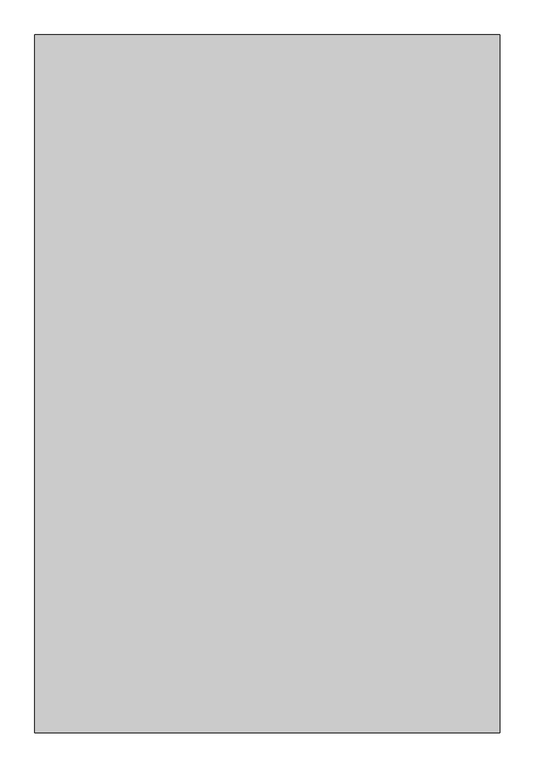
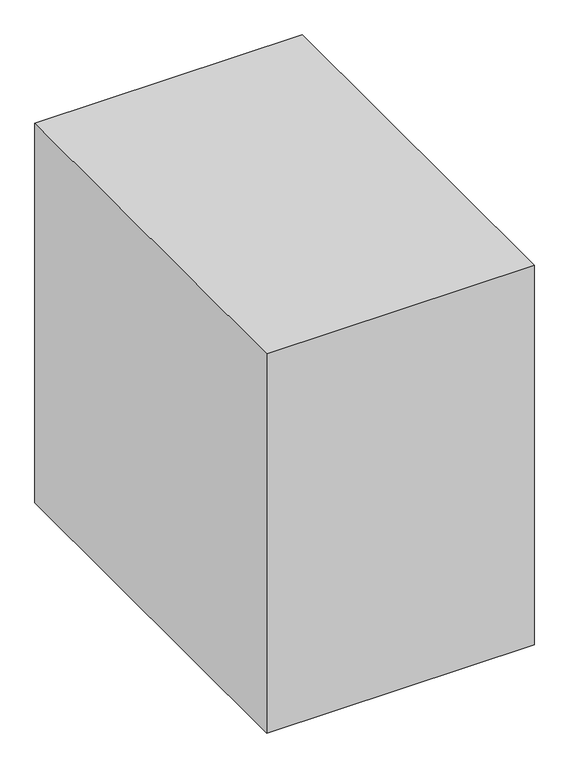
"""IFC4 building model written with IfcOpenShell, lengths in millimetres: proxy geometry, Space Planning Box_hec : Space Planning Box_hec."""

from ifc_helpers import new_model, si_unit, origin, origin_with_axes, place, context, project, spatial, polyline, outline, extrude, source, transform, mapped, element, save


def generic_models_98b71764(model_context):
    return source(origin(), model_context, "Body", "SweptSolid", [
        extrude(outline(polyline([(2000.0, 3000.0), (2000.0, -3000.0), (-2000.0, -3000.0), (-2000.0, 3000.0), (2000.0, 3000.0)])), origin_with_axes(), (0.0, 0.0, 1.0), 6000.0),
    ])


if __name__ == "__main__":
    model = new_model("IFC4")
    model_context = context("Model", 3, world=origin())
    ifc_project = project(units=[si_unit("LENGTHUNIT", "METRE", prefix="MILLI")], contexts=[model_context])
    site = spatial("IfcSite", under=ifc_project)
    building = spatial("IfcBuilding", under=site)
    placement = place(None, origin())
    generic_models_shape = generic_models_98b71764(model_context)
    element("IfcBuildingElementProxy", 1, Name="Space Planning Box_hec : Space Planning Box_hec", ObjectType="Space Planning Box_hec : Space Planning Box_hec", at=placement, inside=building, context=model_context, shape_type="MappedRepresentation", body=[
        mapped(generic_models_shape, transform((0.0, 0.0, 0.0), x_axis=(1.0, 0.0, 0.0), y_axis=(0.0, 1.0, 0.0), z_axis=(0.0, 0.0, 1.0))),
    ])
    save(model, "model.ifc")

# Revit data of these elements
# Type "Space Planning Box_hec : Space Planning Box_hec"
#   Type Comments = "..."
#   Room Name [instance default] = "?"
#   Interior Finish [instance default] = ""
#   Exterior Finish [instance default] = ""
#   Department [instance default] = ""
#   Assembly Code = "..."
#   Width [instance default] = 1524 mm
#   Program Area [instance default] = 0 m²
#   Length [instance default] = 1524 mm
#   Height [instance default] = 1524 mm
#   Area [instance default] = 2.32258 m²
#   Fill Color [instance default] = Cyan
#   Default Elevation = 0
# Element 1 (IfcBuildingElementProxy, "Space Planning Box_hec : Space Planning Box_hec")
#   Room Name = "Shift Office Room"
#   Interior Finish = "IF2-1"
#   Exterior Finish = "EF1"
#   Department = "AR"
#   Width = 4000 mm
#   Program Area = 43.2 m²
#   Length = 6000 mm
#   Height = 6000 mm
#   Area = 24 m²
#   Fill Color = Lavender
#   Materials on its faces: "Lavender"
# Materials
#   "Cyan": class "Generic", colour RGB 0 255 255, transparency 0.2, Cost = 0
#   "Lavender": class "Generic", colour RGB 186 85 211, transparency 0.2, Cost = 0
